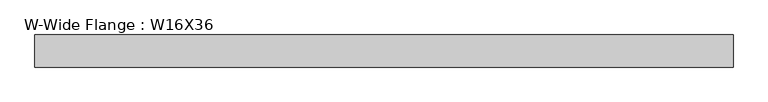
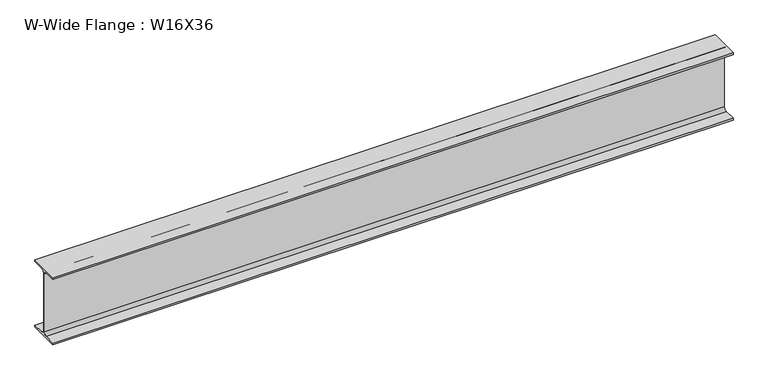
"""IFC4 building model written with IfcOpenShell, lengths in millimetres: beam geometry, W-Wide Flange : W16X36."""

import ifcopenshell
import ifcopenshell.guid

model = None  # the IFC model being written
_history = None  # IfcOwnerHistory: only IFC2X3 demands one
_inside = {}  # id of a spatial element -> (the spatial element, [elements in it])
_under = {}  # id of a project, library or spatial element -> (it, [spatial elements below it])
_declared = {}  # id of a project -> (the project, [libraries it declares])
_typed = {}  # id of a type object -> (the type object, [elements of that type])
_made_of = {}  # id of a material, layer set ... -> (it, [elements and type objects made of it])


def new_model(schema):
    """Start an empty IFC model of exactly this schema.

    Asked for "IFC4X3", IfcOpenShell would pick the latest addendum, in which some entities
    have other attributes; the version numbers below select the first issue.
    IFC2X3 requires an IfcOwnerHistory on every rooted entity: one is made here for all.
    """
    global model, _history
    if schema == "IFC4X3":
        model = ifcopenshell.file(schema_version=(4, 3, 0, 0))
    else:
        model = ifcopenshell.file(schema=schema)
    _inside.clear()
    _under.clear()
    _declared.clear()
    _typed.clear()
    _made_of.clear()
    _history = None
    if model.schema == "IFC2X3":
        org = make("IfcOrganization", Name="unknown")
        user = make(
            "IfcPersonAndOrganization",
            ThePerson=make("IfcPerson", FamilyName="unknown"),
            TheOrganization=org,
        )
        app = make(
            "IfcApplication",
            ApplicationDeveloper=org,
            Version="unknown",
            ApplicationFullName="unknown",
            ApplicationIdentifier="unknown",
        )
        _history = make(
            "IfcOwnerHistory",
            OwningUser=user,
            OwningApplication=app,
            ChangeAction="ADDED",
            CreationDate=0,
        )
    return model


def make(cls, **values):
    """One entity of the class cls with the attributes given. An attribute that is None is left unset."""
    return model.create_entity(
        cls, **{name: value for name, value in values.items() if value is not None}
    )


def rooted(cls, **values):
    """An entity with a GlobalId (a new one), such as an element, a storey or a relation."""
    return make(cls, GlobalId=ifcopenshell.guid.new(), OwnerHistory=_history, **values)


def si_unit(unit_type, name, prefix=None):
    """IfcSIUnit, for example si_unit("LENGTHUNIT", "METRE", prefix="MILLI")."""
    return make("IfcSIUnit", UnitType=unit_type, Prefix=prefix, Name=name)


def assignment(units):
    """IfcUnitAssignment: the units of a project."""
    return None if units is None else make("IfcUnitAssignment", Units=units)


def point(xyz):
    """IfcCartesianPoint."""
    return None if xyz is None else make("IfcCartesianPoint", Coordinates=xyz)


def direction(xyz):
    """IfcDirection."""
    return None if xyz is None else make("IfcDirection", DirectionRatios=xyz)


def frame(location, z_axis=None, x_axis=None):
    """IfcAxis2Placement3D, a coordinate frame: its origin and axes. An axis left out is left unset."""
    return make(
        "IfcAxis2Placement3D",
        Location=point(location),
        Axis=direction(z_axis),
        RefDirection=direction(x_axis),
    )


def frame_2d(location, x_axis=None):
    """IfcAxis2Placement2D, a coordinate frame in the plane: its origin and x axis."""
    return make(
        "IfcAxis2Placement2D", Location=point(location), RefDirection=direction(x_axis)
    )


def origin():
    """The frame at (0, 0, 0) with its axes left unset."""
    return frame((0.0, 0.0, 0.0))


def place(relative_to, where):
    """IfcLocalPlacement: puts the frame where relative to a parent placement (None: the world)."""
    return make(
        "IfcLocalPlacement", PlacementRelTo=relative_to, RelativePlacement=where
    )


def context(
    kind, dimensions, precision=None, world=None, true_north=None, identifier=None
):
    """IfcGeometricRepresentationContext, for example the 3D "Model" context."""
    return make(
        "IfcGeometricRepresentationContext",
        ContextIdentifier=identifier,
        ContextType=kind,
        CoordinateSpaceDimension=dimensions,
        Precision=precision,
        WorldCoordinateSystem=world,
        TrueNorth=true_north,
    )


def project(units=None, contexts=None):
    """IfcProject with its units and contexts."""
    return rooted(
        "IfcProject",
        Name="project",
        RepresentationContexts=contexts,
        UnitsInContext=assignment(units),
    )


def spatial(cls, under=None, at=None, **own):
    """A site, building, storey or space (cls), placed at a placement, below another one or the project."""
    s = rooted(cls, ObjectPlacement=at, **own)
    if under is not None:
        _under.setdefault(under.id(), (under, []))[1].append(s)
    return s


def polyline(points):
    """IfcPolyline through the points."""
    return make("IfcPolyline", Points=[point(p) for p in points])


def circle_curve(where, radius):
    """IfcCircle in the frame where."""
    return make("IfcCircle", Position=where, Radius=radius)


def trimmed(basis, trim1, trim2, sense, master):
    """IfcTrimmedCurve: the piece of a basis curve between two trims."""
    return make(
        "IfcTrimmedCurve",
        BasisCurve=basis,
        Trim1=trim1,
        Trim2=trim2,
        SenseAgreement=sense,
        MasterRepresentation=master,
    )


def segment(curve, same_sense, transition):
    """IfcCompositeCurveSegment."""
    return make(
        "IfcCompositeCurveSegment",
        Transition=transition,
        SameSense=same_sense,
        ParentCurve=curve,
    )


def composite_curve(segments, self_intersect=None):
    """IfcCompositeCurve: segments joined end to end."""
    return make("IfcCompositeCurve", Segments=segments, SelfIntersect=self_intersect)


def outline(outer, holes=None, kind="AREA"):
    """IfcArbitraryClosedProfileDef: a profile drawn as a closed curve; with holes, ...WithVoids."""
    if holes is None:
        return make("IfcArbitraryClosedProfileDef", ProfileType=kind, OuterCurve=outer)
    return make(
        "IfcArbitraryProfileDefWithVoids",
        ProfileType=kind,
        OuterCurve=outer,
        InnerCurves=holes,
    )


def extrude(swept, where, along, depth):
    """IfcExtrudedAreaSolid: the profile swept, set in the frame where, extruded along a direction by depth."""
    return make(
        "IfcExtrudedAreaSolid",
        SweptArea=swept,
        Position=where,
        ExtrudedDirection=direction(along),
        Depth=depth,
    )


def shape(context_of_items, identifier, shape_type, items):
    """IfcShapeRepresentation: the items that make up one representation, for example the "Body"."""
    return make(
        "IfcShapeRepresentation",
        ContextOfItems=context_of_items,
        RepresentationIdentifier=identifier,
        RepresentationType=shape_type,
        Items=items,
    )


def source(mapping_origin, context_of_items, identifier, shape_type, items):
    """IfcRepresentationMap: a shape defined once, which mapped items show again and again."""
    return make(
        "IfcRepresentationMap",
        MappingOrigin=mapping_origin,
        MappedRepresentation=shape(context_of_items, identifier, shape_type, items),
    )


def transform(
    local_origin,
    x_axis=None,
    y_axis=None,
    z_axis=None,
    scale=None,
    scale2=None,
    scale3=None,
    uniform=True,
):
    """IfcCartesianTransformationOperator3D, or its non-uniform kind. x_axis, y_axis, z_axis: its Axis1, 2, 3."""
    if uniform:
        return make(
            "IfcCartesianTransformationOperator3D",
            Axis1=direction(x_axis),
            Axis2=direction(y_axis),
            LocalOrigin=point(local_origin),
            Scale=scale,
            Axis3=direction(z_axis),
        )
    return make(
        "IfcCartesianTransformationOperator3DnonUniform",
        Axis1=direction(x_axis),
        Axis2=direction(y_axis),
        LocalOrigin=point(local_origin),
        Scale=scale,
        Axis3=direction(z_axis),
        Scale2=scale2,
        Scale3=scale3,
    )


def mapped(mapping_source, mapping_target):
    """IfcMappedItem: shows the shape of a source again, moved by a transform."""
    return make(
        "IfcMappedItem", MappingSource=mapping_source, MappingTarget=mapping_target
    )


def made_of(thing, what):
    """Note that an element or type object is made of a material, layer set ...; save() writes the relation."""
    if what is not None:
        _made_of.setdefault(what.id(), (what, []))[1].append(thing)
    return thing


def element(
    cls,
    number,
    at=None,
    inside=None,
    cuts=None,
    type_object=None,
    material=None,
    context=None,
    identifier="Body",
    shape_type=None,
    held_by="IfcProductDefinitionShape",
    body=None,
    shapes=None,
    **own,
):
    """One element of the class cls, such as IfcWall. Its Tag is "e" and its number.

    at: its placement. inside: the storey or other place that contains it. cuts: it is an
    opening in that element (IfcRelVoidsElement). A single representation is given by context,
    identifier, shape_type and body (its items); several are given by shapes. held_by: the class
    of the entity that holds the representations. save() writes the other relations.
    """
    e = rooted(cls, Tag="e%d" % number, ObjectPlacement=at, **own)
    if body is not None:
        shapes = [shape(context, identifier, shape_type, body)]
    if shapes is not None:
        e.Representation = make(held_by, Representations=shapes)
    if inside is not None:
        _inside.setdefault(inside.id(), (inside, []))[1].append(e)
    if cuts is not None:
        rooted(
            "IfcRelVoidsElement", RelatingBuildingElement=cuts, RelatedOpeningElement=e
        )
    if type_object is not None:
        _typed.setdefault(type_object.id(), (type_object, []))[1].append(e)
    return made_of(e, material)


def aggregate(whole, parts):
    """IfcRelAggregates: a whole, such as a stair, and the parts it consists of."""
    return rooted("IfcRelAggregates", RelatingObject=whole, RelatedObjects=parts)


def save(model, path):
    """Write the relations noted so far, then the file.

    IfcRelAggregates (storeys below a building ...), IfcRelContainedInSpatialStructure (elements
    in a storey), IfcRelDefinesByType, IfcRelAssociatesMaterial and IfcRelDeclares: one each for
    every whole, place, type object, material and project.
    """
    for whole, parts in _under.values():
        aggregate(whole, parts)
    for where, things in _inside.values():
        rooted(
            "IfcRelContainedInSpatialStructure",
            RelatedElements=things,
            RelatingStructure=where,
        )
    for kind, things in _typed.values():
        rooted("IfcRelDefinesByType", RelatedObjects=things, RelatingType=kind)
    for what, things in _made_of.values():
        rooted("IfcRelAssociatesMaterial", RelatedObjects=things, RelatingMaterial=what)
    for by, libraries in _declared.values():
        rooted("IfcRelDeclares", RelatingContext=by, RelatedDefinitions=libraries)
    model.write(path)


def w_wide_flange_w16x36_da2d1a7a(model_context):
    return source(origin(), model_context, "Body", "SweptSolid", [
        extrude(outline(composite_curve([segment(polyline([(88.773, -191.008), (88.773, -201.93), (-88.773, -201.93), (-88.773, -191.008), (-21.3995, -191.008)]), True, "CONTINUOUS"), segment(trimmed(circle_curve(frame_2d((-21.3995, -173.355)), 17.653), [point((-21.3995, -191.008))], [point((-3.7465, -173.355))], True, "CARTESIAN"), True, "CONTINUOUS"), segment(polyline([(-3.7465, -173.355), (-3.7465, 173.355)]), True, "CONTINUOUS"), segment(trimmed(circle_curve(frame_2d((-21.3995, 173.355)), 17.653), [point((-3.7465, 173.355))], [point((-21.3995, 191.008))], True, "CARTESIAN"), True, "CONTINUOUS"), segment(polyline([(-21.3995, 191.008), (-88.773, 191.008), (-88.773, 201.93), (88.773, 201.93), (88.773, 191.008), (21.3995, 191.008)]), True, "CONTINUOUS"), segment(trimmed(circle_curve(frame_2d((21.3995, 173.355)), 17.653), [point((21.3995, 191.008))], [point((3.7465, 173.355))], True, "CARTESIAN"), True, "CONTINUOUS"), segment(polyline([(3.7465, 173.355), (3.7465, -173.355)]), True, "CONTINUOUS"), segment(trimmed(circle_curve(frame_2d((21.3995, -173.355)), 17.653), [point((3.7465, -173.355))], [point((21.3995, -191.008))], True, "CARTESIAN"), True, "CONTINUOUS"), segment(polyline([(21.3995, -191.008), (88.773, -191.008)]), True, "CONTINUOUS")], self_intersect=False)), frame((-1893.8875, 0.0, 0.0), z_axis=(1.0, 0.0, 0.0), x_axis=(0.0, 1.0, 0.0)), (0.0, 0.0, 1.0), 3857.6249994),
    ])


if __name__ == "__main__":
    model = new_model("IFC4")
    model_context = context("Model", 3, world=origin())
    ifc_project = project(units=[si_unit("LENGTHUNIT", "METRE", prefix="MILLI")], contexts=[model_context])
    site = spatial("IfcSite", under=ifc_project)
    building = spatial("IfcBuilding", under=site)
    placement = place(None, origin())
    w_wide_flange_w16x36_shape = w_wide_flange_w16x36_da2d1a7a(model_context)
    element("IfcBeam", 1, ObjectType="W-Wide Flange : W16X36", at=placement, inside=building, context=model_context, shape_type="MappedRepresentation", body=[
        mapped(w_wide_flange_w16x36_shape, transform((0.0, 0.0, 0.0), x_axis=(1.0, 0.0, 0.0), y_axis=(0.0, 1.0, 0.0), z_axis=(0.0, 0.0, 1.0))),
    ])
    save(model, "model.ifc")

# Revit data of these elements
# Type "W-Wide Flange : W16X36"
#   Assembly Code = "B10"
#   W = 36
#   Length [instance default] = 5' - 0"
#   bf = 0' - 6.99"
#   d = 1' - 3.9"
#   k = 0' - 1 1/8"
#   k2 = 0' - 0.695"
#   tf = 0' - 0.43"
#   tw = 0' - 0.295"
#   A = 0.0736111 SF
#   Structural Material [instance default] = Steel ASTM A992
# Element 1 (IfcBeam, "W-Wide Flange : W16X36")
#   Materials on its faces: "Steel ASTM A992"
# Materials
#   "Steel ASTM A992": class "Metal", colour RGB 199 199 199, transparency 0, Description = "Structural steel 50ksi", Cost = 0
